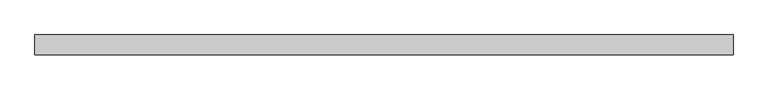
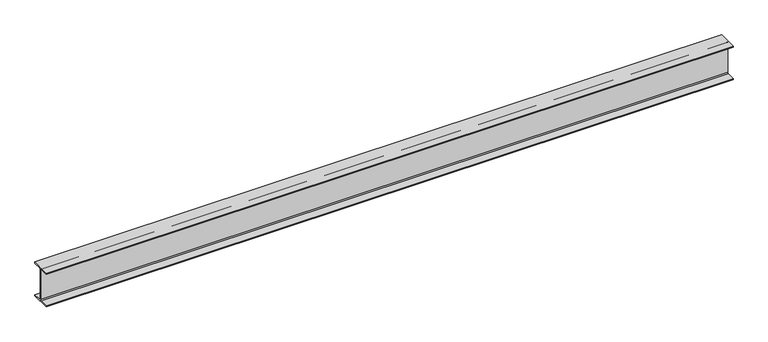
"""IFC4 building model written with IfcOpenShell, lengths in millimetres: beam geometry, Old_Steel Beam_H-KSD3502 : H_SB_ASB_H-200×200x8x12."""

from ifc_helpers import new_model, si_unit, point, frame, frame_2d, origin, place, context, project, spatial, polyline, circle_curve, trimmed, segment, composite_curve, outline, extrude, source, transform, mapped, element, save


def beam_0b84e835(model_context):
    return source(origin(), model_context, "Body", "SweptSolid", [
        extrude(outline(composite_curve([segment(polyline([(82.5, -141.5), (82.5, -151.7), (-82.5, -151.7), (-82.5, -141.5), (-11.9, -141.5)]), True, "CONTINUOUS"), segment(trimmed(circle_curve(frame_2d((-11.9, -132.6)), 8.9), [point((-11.9, -141.5))], [point((-3.0, -132.6))], True, "CARTESIAN"), True, "CONTINUOUS"), segment(polyline([(-3.0, -132.6), (-3.0, 132.6)]), True, "CONTINUOUS"), segment(trimmed(circle_curve(frame_2d((-11.9, 132.6)), 8.9), [point((-3.0, 132.6))], [point((-11.9, 141.5))], True, "CARTESIAN"), True, "CONTINUOUS"), segment(polyline([(-11.9, 141.5), (-82.5, 141.5), (-82.5, 151.7), (82.5, 151.7), (82.5, 141.5), (11.9, 141.5)]), True, "CONTINUOUS"), segment(trimmed(circle_curve(frame_2d((11.9, 132.6)), 8.9), [point((11.9, 141.5))], [point((3.0, 132.6))], True, "CARTESIAN"), True, "CONTINUOUS"), segment(polyline([(3.0, 132.6), (3.0, -132.6)]), True, "CONTINUOUS"), segment(trimmed(circle_curve(frame_2d((11.9, -132.6)), 8.9), [point((3.0, -132.6))], [point((11.9, -141.5))], True, "CARTESIAN"), True, "CONTINUOUS"), segment(polyline([(11.9, -141.5), (82.5, -141.5)]), True, "CONTINUOUS")], self_intersect=False)), frame((-3120.023728, 0.0, 0.0), z_axis=(1.0, 0.0, 0.0), x_axis=(0.0, 1.0, 0.0)), (0.0, 0.0, 1.0), 5840.8278571),
    ])


if __name__ == "__main__":
    model = new_model("IFC4")
    model_context = context("Model", 3, world=origin())
    ifc_project = project(units=[si_unit("LENGTHUNIT", "METRE", prefix="MILLI")], contexts=[model_context])
    site = spatial("IfcSite", under=ifc_project)
    building = spatial("IfcBuilding", under=site)
    placement = place(None, origin())
    beam_shape = beam_0b84e835(model_context)
    element("IfcBeam", 1, ObjectType="Old_Steel Beam_H-KSD3502 : H_SB_ASB_H-200×200x8x12", at=placement, inside=building, context=model_context, shape_type="MappedRepresentation", body=[
        mapped(beam_shape, transform((0.0, 0.0, 0.0), x_axis=(1.0, 0.0, 0.0), y_axis=(0.0, 1.0, 0.0), z_axis=(0.0, 0.0, 1.0))),
    ])
    save(model, "model.ifc")

# Revit data of these elements
# Type "Old_Steel Beam_H-KSD3502 : H_SB_ASB_H-200×200x8x12"
#   Width = 20.0 cm
#   Web Thickness = 0.8 cm
#   Web Fillet = 1.3 cm
#   Warping Constant = 141376.0 cm⁶
#   Torsional Moment of Inertia = 26.2485 cm⁴
#   Torsional Modulus = 1.0 cm³
#   Section Area = 63.53 cm²
#   Plastic Modulus weak axis = 244.0 cm³
#   Plastic Modulus strong axis = 525.0 cm³
#   Perimeter = 1.16 m²/m
#   Nominal Weight = 49.90 kgf/m
#   Moment of Inertia weak axis = 1600.00 cm⁴
#   Moment of Inertia strong axis = 4720.00 cm⁴
#   Height = 20.0 cm
#   Flange Thickness = 1.2 cm
#   Elastic Modulus weak axis = 160.0 cm³
#   Elastic Modulus strong axis = 472.0 cm³
#   Centroid Vertical = 10.0 cm
#   Centroid Horizontal = 10.0 cm
#   Length [instance default] = 1.5240 m
#   Structural Material [instance default] = Steel, 45-345
#   Assembly Code = ""
# Element 1 (IfcBeam, "Old_Steel Beam_H-KSD3502 : H_SB_ASB_H-200×200x8x12")
#   Structural Material = none
# Materials
#   "Steel, 45-345": class "Metal", colour RGB 189 187 185, transparency 0, Description = "Steel 345 MPa", Cost = 0
